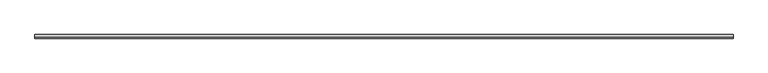
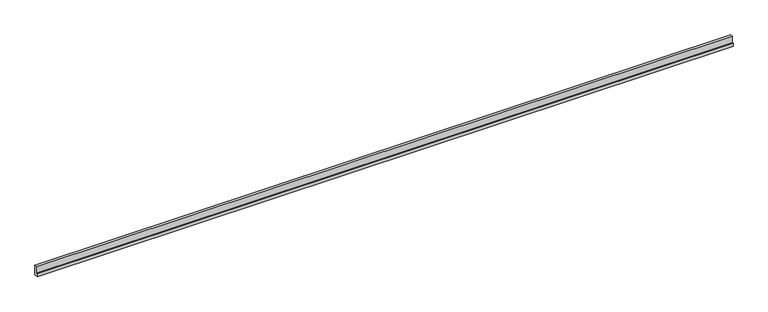
"""IFC4 building model written with IfcOpenShell, lengths in millimetres: proxy geometry, Generic Models 7:Generic Models 1:337419:Generic Models 1:337419 : Generic Models 7:Generic Models 1:337419:16 : Generic Models 7:Generic Models 1:337419:Generic Models 1:337419 : Generic Models 7:Generic Models 1:337419:301336."""

from ifc_helpers import new_model, si_unit, frame, origin, place, context, project, spatial, polyline, outline, extrude, source, transform, mapped, element, save


def generic_models_5cc94d66(model_context):
    return source(origin(), model_context, "Body", "SweptSolid", [
        extrude(outline(polyline([(-536547.61719, 8523.6954936), (-536547.61719, 8571.6070313), (-536531.8913358, 8571.6070313), (-536531.8913358, 8502.1984758), (-536557.2913358, 8502.1984758), (-536557.2913358, 8523.6954936), (-536547.61719, 8523.6954936)])), frame((591306.0367242, 0.0, 0.0), z_axis=(1.0, 0.0, 0.0), x_axis=(0.0, 1.0, 0.0)), (0.0, 0.0, 1.0), 4876.8),
    ])


if __name__ == "__main__":
    model = new_model("IFC4")
    model_context = context("Model", 3, world=origin())
    ifc_project = project(units=[si_unit("LENGTHUNIT", "METRE", prefix="MILLI")], contexts=[model_context])
    site = spatial("IfcSite", under=ifc_project)
    building = spatial("IfcBuilding", under=site)
    placement = place(None, origin())
    generic_models_shape = generic_models_5cc94d66(model_context)
    element("IfcBuildingElementProxy", 1, Name="Generic Models 7:Generic Models 1:337419:Generic Models 1:337419 : Generic Models 7:Generic Models 1:337419:16 : Generic Models 7:Generic Models 1:337419:Generic Models 1:337419 : Generic Models 7:Generic Models 1:337419:301336", ObjectType="Generic Models 7:Generic Models 1:337419:Generic Models 1:337419 : Generic Models 7:Generic Models 1:337419:16 : Generic Models 7:Generic Models 1:337419:Generic Models 1:337419 : Generic Models 7:Generic Models 1:337419:301336", at=placement, inside=building, context=model_context, shape_type="MappedRepresentation", body=[
        mapped(generic_models_shape, transform((0.0, 0.0, 0.0), x_axis=(1.0, 0.0, 0.0), y_axis=(0.0, 1.0, 0.0), z_axis=(0.0, 0.0, 1.0))),
    ])
    save(model, "model.ifc")

# Revit data of these elements
# Type "Generic Models 7:Generic Models 1:337419:Generic Models 1:337419 : Generic Models 7:Generic Models 1:337419:16 : Generic Models 7:Generic Models 1:337419:Generic Models 1:337419 : Generic Models 7:Generic Models 1:337419:301336"
#   NameOverride = "Generic Models 7:Generic Models 1:337419:Generic Models 1:337419 : Generic Models 7:Generic Models 1:337419:301336"
#   ObjectTypeOverride = "Generic Models 1:337419 : Generic Models 7:Generic Models 1:337419"
#   Reference = "Generic Models 1"
#   Tag = "301336"
# Element 1 (IfcBuildingElementProxy, "Generic Models 7:Generic Models 1:337419:Generic Models 1:337419 : Generic Models 7:Generic Models 1:337419:16 : Generic Models 7:Generic Models 1:337419:Generic Models 1:337419 : Generic Models 7:Generic Models 1:337419:301336")
#   Materials on its faces: "RIGID INSULATION AT GIRTS/JAMB - (CLASS A FLAME SPREAD)"
# Materials
#   "RIGID INSULATION AT GIRTS/JAMB - (CLASS A FLAME SPREAD)": class "Unassigned", colour RGB 205 188 106, transparency 0, Cost = 0
